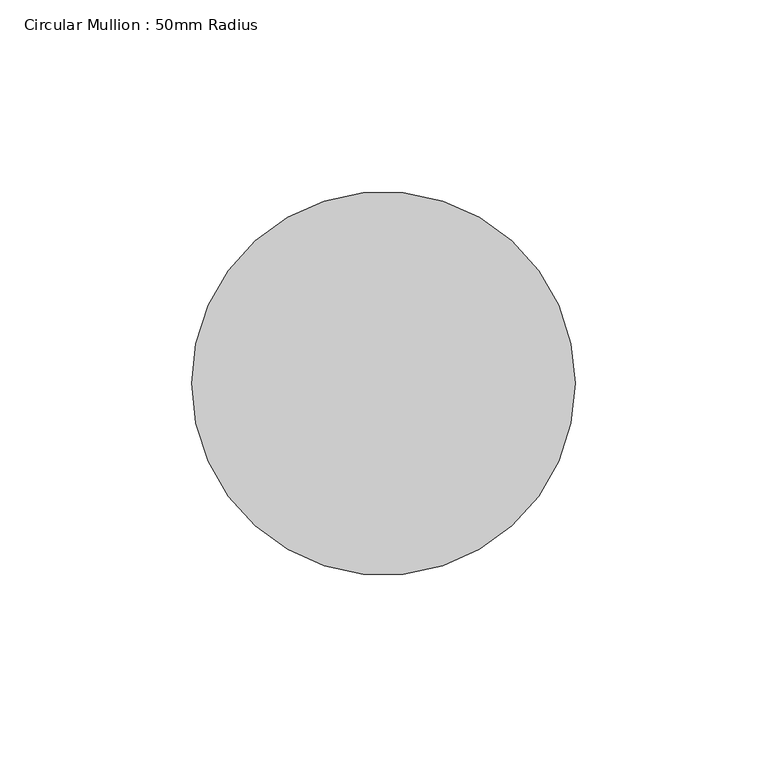
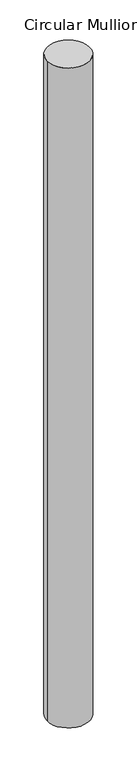
"""IFC4 building model written with IfcOpenShell, lengths in millimetres: member geometry, Circular Mullion : 50mm Radius."""

from ifc_helpers import new_model, si_unit, point, frame, origin, origin_2d, place, context, project, spatial, circle_curve, trimmed, segment, composite_curve, outline, extrude, source, transform, mapped, element, save


def circular_mullion_50mm_radius_b9333bcc(model_context):
    return source(origin(), model_context, "Body", "SweptSolid", [
        extrude(outline(composite_curve([segment(trimmed(circle_curve(origin_2d(), 50.0), [point((50.0, 0.0))], [point((-50.0, 0.0))], False, "CARTESIAN"), True, "CONTINUOUS"), segment(trimmed(circle_curve(origin_2d(), 50.0), [point((-50.0, 0.0))], [point((50.0, 0.0))], False, "CARTESIAN"), True, "CONTINUOUS")], self_intersect=False)), frame((0.0, 0.0, -1648.3387721), z_axis=(0.0, 0.0, 1.0), x_axis=(1.0, 0.0, 0.0)), (0.0, 0.0, 1.0), 1648.3387721),
    ])


if __name__ == "__main__":
    model = new_model("IFC4")
    model_context = context("Model", 3, world=origin())
    ifc_project = project(units=[si_unit("LENGTHUNIT", "METRE", prefix="MILLI")], contexts=[model_context])
    site = spatial("IfcSite", under=ifc_project)
    building = spatial("IfcBuilding", under=site)
    placement = place(None, origin())
    circular_mullion_50mm_radius_shape = circular_mullion_50mm_radius_b9333bcc(model_context)
    element("IfcMember", 1, ObjectType="Circular Mullion : 50mm Radius", at=placement, inside=building, context=model_context, shape_type="MappedRepresentation", body=[
        mapped(circular_mullion_50mm_radius_shape, transform((0.0, 0.0, 0.0), x_axis=(1.0, 0.0, 0.0), y_axis=(0.0, 1.0, 0.0), z_axis=(0.0, 0.0, 1.0))),
    ])
    save(model, "model.ifc")

# Revit data of these elements
# Type "Circular Mullion : 50mm Radius"
#   built-in parameter 1007350 = 0.164042 (stored number, unit not read)
# Element 1 (IfcMember, "Circular Mullion : 50mm Radius")
#   Materials on its faces: "Aluminium"
# Materials
#   "Aluminium": class "Metal", colour RGB 247 247 247, transparency 0, Description = "Aluminium 6061", Cost = 0
